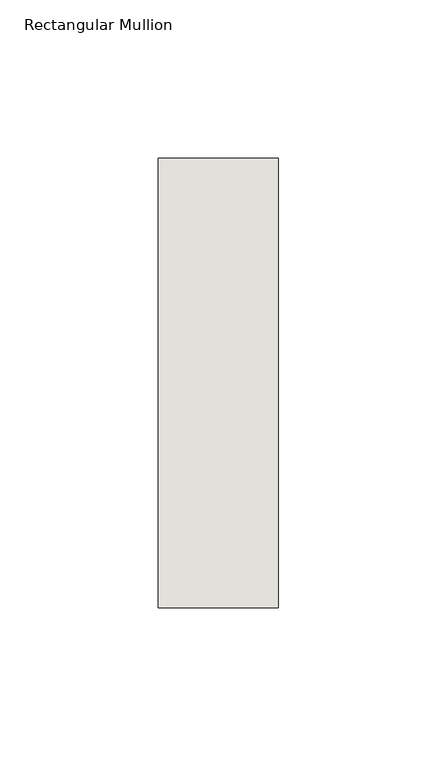
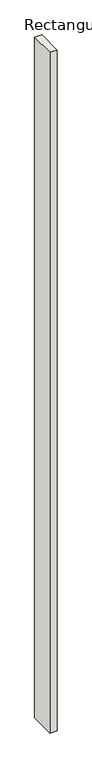
"""IFC4 building model written with IfcOpenShell, lengths in millimetres: wall geometry, Rectangular Mullion : NLRS_21_CWM_hsb-regel 38x142_gen_rsf."""

from ifc_helpers import new_model, si_unit, frame, origin, place, context, project, spatial, polyline, outline, extrude, source, transform, mapped, element, save


def rectangular_mullion_f62802ff(model_context):
    return source(origin(), model_context, "Body", "SweptSolid", [
        extrude(outline(polyline([(0.0, -71.0), (-38.0, -71.0), (-38.0, 71.0), (0.0, 71.0), (0.0, -71.0)])), frame((0.0, 0.0, -3849.0), z_axis=(0.0, 0.0, 1.0), x_axis=(1.0, 0.0, 0.0)), (0.0, 0.0, 1.0), 3849.0),
    ])


if __name__ == "__main__":
    model = new_model("IFC4")
    model_context = context("Model", 3, world=origin())
    ifc_project = project(units=[si_unit("LENGTHUNIT", "METRE", prefix="MILLI")], contexts=[model_context])
    site = spatial("IfcSite", under=ifc_project)
    building = spatial("IfcBuilding", under=site)
    placement = place(None, origin())
    rectangular_mullion_shape = rectangular_mullion_f62802ff(model_context)
    element("IfcWall", 1, ObjectType="Rectangular Mullion : NLRS_21_CWM_hsb-regel 38x142_gen_rsf", at=placement, inside=building, context=model_context, shape_type="MappedRepresentation", body=[
        mapped(rectangular_mullion_shape, transform((0.0, 0.0, 0.0), x_axis=(1.0, 0.0, 0.0), y_axis=(0.0, 1.0, 0.0), z_axis=(0.0, 0.0, 1.0))),
    ])
    save(model, "model.ifc")

# Revit data of these elements
# Type "Rectangular Mullion : NLRS_21_CWM_hsb-regel 38x142_gen_rsf"
#   Type IfcGUID = "07M7mRoiH1CR8m_RSKIwpF"
#   Assembly Code = "21.10"
#   IfcExportAs = "IfcWall"
#   built-in parameter 1007322 = 0.465879 (stored number, unit not read)
#   built-in parameter 1007321 = 0.062336 (stored number, unit not read)
#   built-in parameter 1007320 = 0.062336 (stored number, unit not read)
# Element 1 (IfcWall, "Rectangular Mullion : NLRS_21_CWM_hsb-regel 38x142_gen_rsf")
#   Materials on its faces: "NLRS_i2_hout naaldhout vuren_gen_rsf"
# Materials
#   "NLRS_i2_hout naaldhout vuren_gen_rsf": class "I - Hout", colour RGB 234 199 147, transparency 0, Keynote = "i2", Manufacturer = "Revit Standards Foundation", URL = "www.revitstandards.org", Description = "hout vuren", Cost = 0
